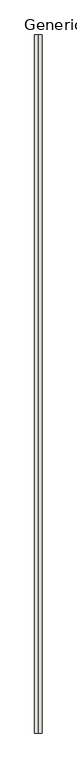
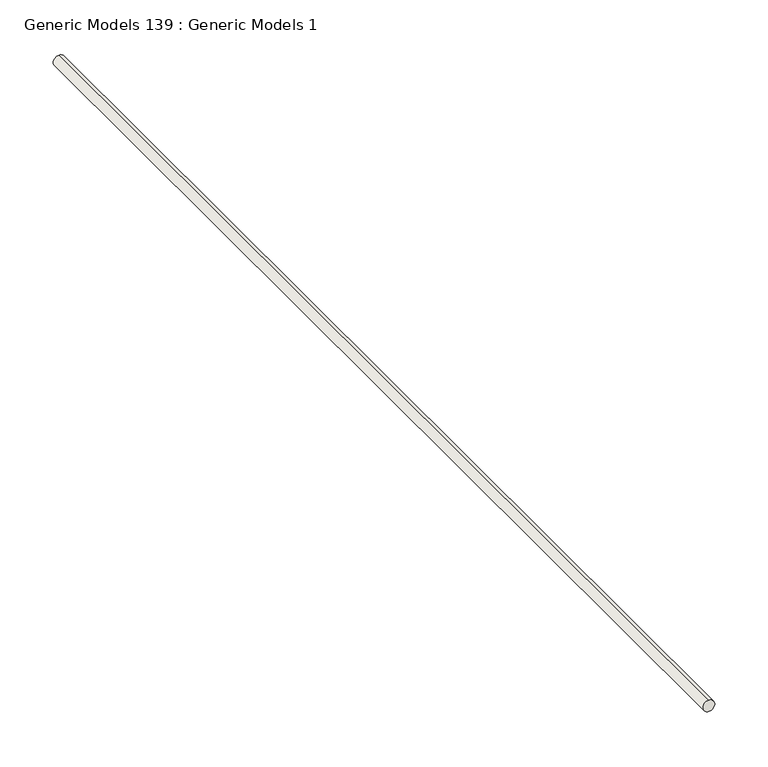
"""IFC4 building model written with IfcOpenShell, lengths in millimetres: wall geometry, Generic Models 139 : Generic Models 1."""

from ifc_helpers import new_model, si_unit, point, frame, frame_2d, origin, place, context, project, spatial, circle_curve, trimmed, segment, composite_curve, outline, extrude, source, transform, mapped, element, save


def generic_models_139_generic_models_1_dcce0395(model_context):
    return source(origin(), model_context, "Body", "SweptSolid", [
        extrude(outline(composite_curve([segment(trimmed(circle_curve(frame_2d((-76.2, 51947.7625)), 6.35), [point((-82.55, 51947.7625))], [point((-69.85, 51947.7625))], False, "CARTESIAN"), True, "CONTINUOUS"), segment(trimmed(circle_curve(frame_2d((-76.2, 51947.7625)), 6.35), [point((-69.85, 51947.7625))], [point((-82.55, 51947.7625))], False, "CARTESIAN"), True, "CONTINUOUS")], self_intersect=False)), frame((0.0, 0.0, 0.0), z_axis=(0.0, 1.0, 0.0), x_axis=(0.0, 0.0, 1.0)), (0.0, 0.0, 1.0), 1219.2),
    ])


if __name__ == "__main__":
    model = new_model("IFC4")
    model_context = context("Model", 3, world=origin())
    ifc_project = project(units=[si_unit("LENGTHUNIT", "METRE", prefix="MILLI")], contexts=[model_context])
    site = spatial("IfcSite", under=ifc_project)
    building = spatial("IfcBuilding", under=site)
    placement = place(None, origin())
    generic_models_139_generic_models_1_shape = generic_models_139_generic_models_1_dcce0395(model_context)
    element("IfcWall", 1, ObjectType="Generic Models 139 : Generic Models 1", at=placement, inside=building, context=model_context, shape_type="MappedRepresentation", body=[
        mapped(generic_models_139_generic_models_1_shape, transform((0.0, 0.0, 0.0), x_axis=(1.0, 0.0, 0.0), y_axis=(0.0, 1.0, 0.0), z_axis=(0.0, 0.0, 1.0))),
    ])
    save(model, "model.ifc")

# Revit data of these elements
# Element 1 (IfcWall, "Generic Models 139 : Generic Models 1")
#   Materials on its faces: "#4 CONT. STEEL REBAR"
# Materials
#   "#4 CONT. STEEL REBAR": class "Metal", colour RGB 189 187 185, transparency 0, Description = "Structural steel 50ksi", Cost = 0
